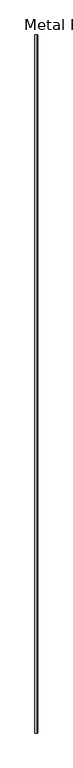
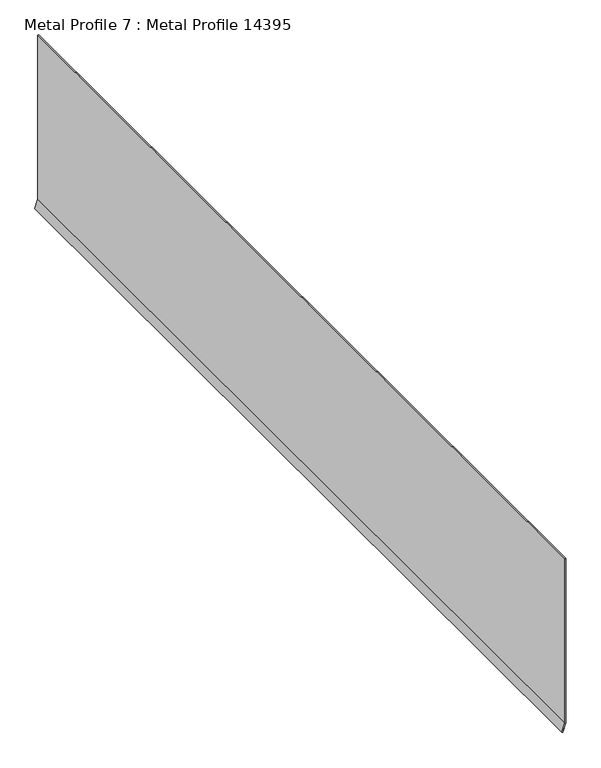
"""IFC4 building model written with IfcOpenShell, lengths in millimetres: proxy geometry, Metal Profile 7 : Metal Profile 14395."""

from ifc_helpers import new_model, si_unit, frame, origin, place, context, project, spatial, polyline, outline, extrude, source, transform, mapped, element, save


def metal_profile_7_metal_profile_14395_face8f0a(model_context):
    return source(origin(), model_context, "Body", "SweptSolid", [
        extrude(outline(polyline([(44076.0101511, 5319.4569239), (44076.0101511, 5317.4569239), (43696.0101511, 5317.4569239), (43676.3589507, 5311.0919258), (43675.7426741, 5312.994609), (43695.6943291, 5319.4569239), (44076.0101511, 5319.4569239)])), frame((0.0, -1830.9378034, 0.0), z_axis=(0.0, 1.0, 0.0), x_axis=(0.0, 0.0, 1.0)), (0.0, 0.0, 1.0), 1999.85),
    ])


if __name__ == "__main__":
    model = new_model("IFC4")
    model_context = context("Model", 3, world=origin())
    ifc_project = project(units=[si_unit("LENGTHUNIT", "METRE", prefix="MILLI")], contexts=[model_context])
    site = spatial("IfcSite", under=ifc_project)
    building = spatial("IfcBuilding", under=site)
    placement = place(None, origin())
    metal_profile_7_metal_profile_14395_shape = metal_profile_7_metal_profile_14395_face8f0a(model_context)
    element("IfcBuildingElementProxy", 1, Name="Metal Profile 7 : Metal Profile 14395", ObjectType="Metal Profile 7 : Metal Profile 14395", at=placement, inside=building, context=model_context, shape_type="MappedRepresentation", body=[
        mapped(metal_profile_7_metal_profile_14395_shape, transform((0.0, 0.0, 0.0), x_axis=(1.0, 0.0, 0.0), y_axis=(0.0, 1.0, 0.0), z_axis=(0.0, 0.0, 1.0))),
    ])
    save(model, "model.ifc")

# Revit data of these elements
# Type "Metal Profile 7 : Metal Profile 14395"
#   NameOverride = "Metal Profile"
# Element 1 (IfcBuildingElementProxy, "Metal Profile 7 : Metal Profile 14395")
#   Materials on its faces: "20 GA. CONTINUOUS CLEAT"
# Materials
#   "20 GA. CONTINUOUS CLEAT": class "Unassigned", colour RGB 245 226 176, transparency 0, Cost = 0
